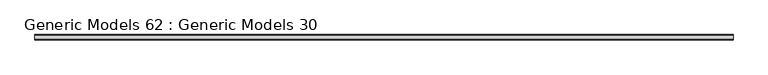
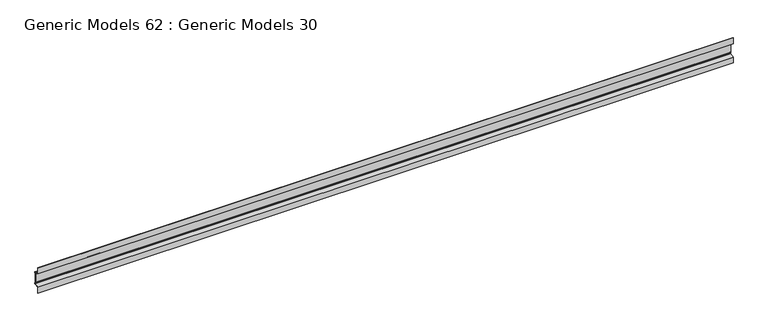
"""IFC4 building model written with IfcOpenShell, lengths in millimetres: proxy geometry, Generic Models 62 : Generic Models 30."""

from ifc_helpers import new_model, si_unit, point, frame, frame_2d, origin, place, context, project, spatial, polyline, circle_curve, trimmed, segment, composite_curve, outline, extrude, source, transform, mapped, element, save


def generic_models_62_generic_models_30_4e927001(model_context):
    return source(origin(), model_context, "Body", "SweptSolid", [
        extrude(outline(composite_curve([segment(polyline([(40961.0137657, 268832.7746691), (40970.2579, 268830.7357718)]), True, "CONTINUOUS"), segment(trimmed(circle_curve(frame_2d((40969.7450157, 268828.4104114)), 2.38125), [point((40970.2579, 268830.7357718))], [point((40971.3325157, 268826.6355324))], False, "CARTESIAN"), True, "CONTINUOUS"), segment(trimmed(circle_curve(frame_2d((40972.9200157, 268824.8606535)), 2.38125), [point((40971.3325157, 268826.6355324))], [point((40970.5387657, 268824.8606535))], True, "CARTESIAN"), True, "CONTINUOUS"), segment(polyline([(40970.5387657, 268824.8606535), (40970.5387657, 268804.2393465)]), True, "CONTINUOUS"), segment(trimmed(circle_curve(frame_2d((40972.9200157, 268804.2393465)), 2.38125), [point((40970.5387657, 268804.2393465))], [point((40971.3325157, 268802.4644676))], True, "CARTESIAN"), True, "CONTINUOUS"), segment(trimmed(circle_curve(frame_2d((40969.7450157, 268800.6895886)), 2.38125), [point((40971.3325157, 268802.4644676))], [point((40970.2579, 268798.3642282))], False, "CARTESIAN"), True, "CONTINUOUS"), segment(polyline([(40970.2579, 268798.3642282), (40961.0137657, 268796.3253309), (40961.0137657, 268782.8), (40959.4262657, 268782.8), (40959.4262657, 268797.6008453), (40969.9159772, 268799.9144685)]), True, "CONTINUOUS"), segment(trimmed(circle_curve(frame_2d((40969.7450157, 268800.6895886)), 0.79375), [point((40969.9159772, 268799.9144685))], [point((40970.2741824, 268801.2812149))], True, "CARTESIAN"), True, "CONTINUOUS"), segment(trimmed(circle_curve(frame_2d((40972.9200157, 268804.2393465)), 3.96875), [point((40970.2741824, 268801.2812149))], [point((40968.9512657, 268804.2393465))], False, "CARTESIAN"), True, "CONTINUOUS"), segment(polyline([(40968.9512657, 268804.2393465), (40968.9512657, 268824.8606535)]), True, "CONTINUOUS"), segment(trimmed(circle_curve(frame_2d((40972.9200157, 268824.8606535)), 3.96875), [point((40968.9512657, 268824.8606535))], [point((40970.2741824, 268827.8187851))], False, "CARTESIAN"), True, "CONTINUOUS"), segment(trimmed(circle_curve(frame_2d((40969.7450157, 268828.4104114)), 0.79375), [point((40970.2741824, 268827.8187851))], [point((40969.9159772, 268829.1855315))], True, "CARTESIAN"), True, "CONTINUOUS"), segment(polyline([(40969.9159772, 268829.1855315), (40959.4262657, 268831.4991547), (40959.4262657, 268846.3), (40961.0137657, 268846.3), (40961.0137657, 268832.7746691)]), True, "CONTINUOUS")], self_intersect=False)), frame((26427.4962986, 0.0, 0.0), z_axis=(1.0, 0.0, 0.0), x_axis=(0.0, 1.0, 0.0)), (0.0, 0.0, 1.0), 1676.4),
    ])


if __name__ == "__main__":
    model = new_model("IFC4")
    model_context = context("Model", 3, world=origin())
    ifc_project = project(units=[si_unit("LENGTHUNIT", "METRE", prefix="MILLI")], contexts=[model_context])
    site = spatial("IfcSite", under=ifc_project)
    building = spatial("IfcBuilding", under=site)
    placement = place(None, origin())
    generic_models_62_generic_models_30_shape = generic_models_62_generic_models_30_4e927001(model_context)
    element("IfcBuildingElementProxy", 1, Name="Generic Models 62 : Generic Models 30", ObjectType="Generic Models 62 : Generic Models 30", at=placement, inside=building, context=model_context, shape_type="MappedRepresentation", body=[
        mapped(generic_models_62_generic_models_30_shape, transform((0.0, 0.0, 0.0), x_axis=(1.0, 0.0, 0.0), y_axis=(0.0, 1.0, 0.0), z_axis=(0.0, 0.0, 1.0))),
    ])
    save(model, "model.ifc")

# Revit data of these elements
# Element 1 (IfcBuildingElementProxy, "Generic Models 62 : Generic Models 30")
#   Materials on its faces: "1/2\" DEEP GALV. HORTZ. HAT CHANNEL @ XX O.C."
# Materials
#   "1/2\" DEEP GALV. HORTZ. HAT CHANNEL @ XX O.C.": class "Generic", colour RGB 212 212 212, transparency 0, Cost = 0
